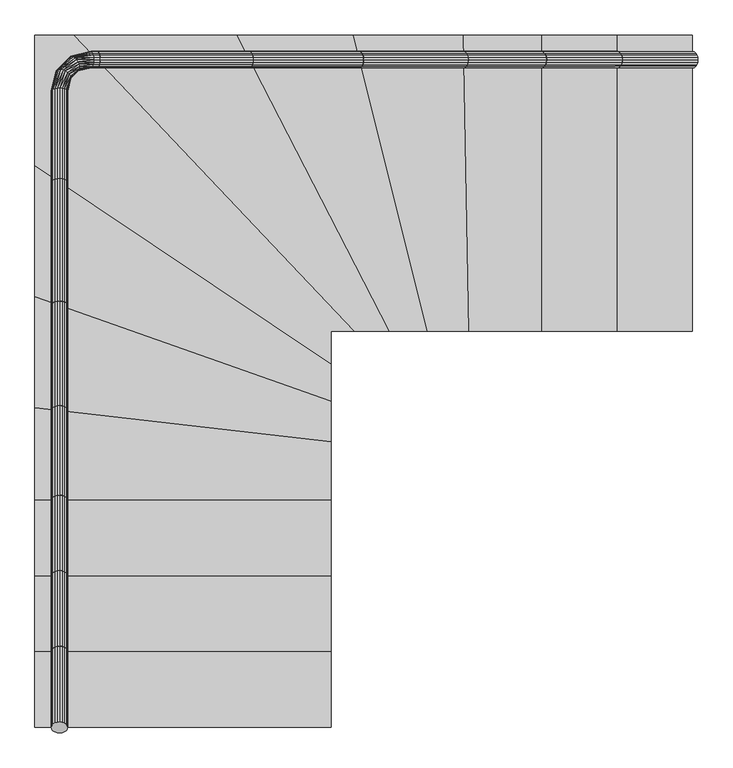
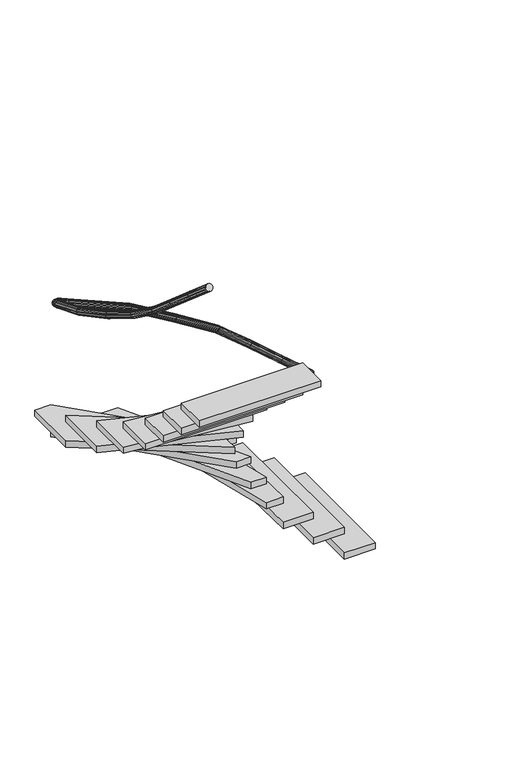
"""IFC4 building model written with IfcOpenShell, lengths in millimetres: stair geometry, 0_3d_modell."""

from ifc_helpers import new_model, si_unit, frame, origin, origin_with_axes, place, context, project, spatial, polyline, outline, extrude, faceted_brep, source, transform, mapped, element, save


def stair_ec7f74a5(model_context):
    return source(origin(), model_context, "Body", "SolidModel", [
        faceted_brep([(51.2235871, 975.7637439, 2650.066583), (50.0, 980.2280824, 2656.7020937), (51.2235871, 984.692421, 2663.3376045), (54.7745751, 988.719759, 2669.3235852), (60.3053687, 991.9158725, 2674.0740863), (67.2745751, 993.9679037, 2677.1240958), (75.0, 994.6749855, 2678.1750575), (82.7254249, 993.9679037, 2677.1240958), (89.6946313, 991.9158725, 2674.0740863), (95.2254249, 988.719759, 2669.3235852), (98.7764129, 984.692421, 2663.3376045), (100.0, 980.2280824, 2656.7020937), (98.7764129, 975.7637439, 2650.066583), (95.2254249, 971.7364059, 2644.0806023), (89.6946313, 968.5402924, 2639.3301012), (82.7254249, 966.4882612, 2636.2800917), (75.0, 965.7811794, 2635.22913), (67.2745751, 966.4882612, 2636.2800917), (60.3053687, 968.5402924, 2639.3301012), (54.7745751, 971.7364059, 2644.0806023), (51.2235871, 711.8708742, 2861.5423857), (50.0, 706.9018591, 2855.2735223), (51.2235871, 701.932844, 2849.004659), (54.7745751, 697.4502308, 2843.3494356), (60.3053687, 693.8928087, 2838.861425), (67.2745751, 691.6088032, 2835.9799448), (75.0, 690.8217885, 2834.9870544), (82.7254249, 691.6088032, 2835.9799448), (89.6946313, 693.8928087, 2838.861425), (95.2254249, 697.4502308, 2843.3494356), (98.7764129, 701.932844, 2849.004659), (100.0, 706.9018591, 2855.2735223), (98.7764129, 711.8708742, 2861.5423857), (95.2254249, 716.3534875, 2867.197609), (89.6946313, 719.9109095, 2871.6856196), (82.7254249, 722.194915, 2874.5670998), (75.0, 722.9819297, 2875.5599903), (67.2745751, 722.194915, 2874.5670998), (60.3053687, 719.9109095, 2871.6856196), (54.7745751, 716.3534875, 2867.197609)], [[[0, 1, 2, 3, 4, 5, 6, 7, 8, 9, 10, 11, 12, 13, 14, 15, 16, 17, 18, 19]], [[20, 21, 22, 23, 24, 25, 26, 27, 28, 29, 30, 31, 32, 33, 34, 35, 36, 37, 38, 39]], [[2, 1, 21, 20]], [[3, 2, 20, 39]], [[4, 3, 39, 38]], [[5, 4, 38, 37]], [[6, 5, 37, 36]], [[7, 6, 36, 35]], [[8, 7, 35, 34]], [[9, 8, 34, 33]], [[10, 9, 33, 32]], [[11, 10, 32, 31]], [[12, 11, 31, 30]], [[13, 12, 30, 29]], [[14, 13, 29, 28]], [[15, 14, 28, 27]], [[16, 15, 27, 26]], [[17, 16, 26, 25]], [[18, 17, 25, 24]], [[19, 18, 24, 23]], [[0, 19, 23, 22]], [[1, 0, 22, 21]]]),
        extrude(outline(polyline([(970.0, 1221.5036957), (900.0, 1221.5036957), (900.0, 1121.5036957), (0.0, 1724.0707938), (0.0, 2121.5036957), (118.0988626, 2121.5036957), (970.0, 1221.5036957)])), frame((0.0, 0.0, 1191.4285714), z_axis=(0.0, 0.0, 1.0), x_axis=(1.0, 0.0, 0.0)), (0.0, 0.0, 1.0), 50.0),
        faceted_brep([(51.2235871, 701.932844, 2849.004659), (50.0, 706.9018591, 2855.2735223), (51.2235871, 711.8708742, 2861.5423857), (54.7745751, 716.3534875, 2867.197609), (60.3053687, 719.9109095, 2871.6856196), (67.2745751, 722.194915, 2874.5670998), (75.0, 722.9819297, 2875.5599903), (82.7254249, 722.194915, 2874.5670998), (89.6946313, 719.9109095, 2871.6856196), (95.2254249, 716.3534875, 2867.197609), (98.7764129, 711.8708742, 2861.5423857), (100.0, 706.9018591, 2855.2735223), (98.7764129, 701.932844, 2849.004659), (95.2254249, 697.4502308, 2843.3494356), (89.6946313, 693.8928087, 2838.861425), (82.7254249, 691.6088032, 2835.9799448), (75.0, 690.8217885, 2834.9870544), (67.2745751, 691.6088032, 2835.9799448), (60.3053687, 693.8928087, 2838.861425), (54.7745751, 697.4502308, 2843.3494356), (51.2235871, 482.1248208, 3059.8945684), (50.0, 476.9018591, 3053.8449509), (51.2235871, 471.6788974, 3047.7953334), (54.7745751, 466.9671956, 3042.3378946), (60.3053687, 463.2279679, 3038.0068466), (67.2745751, 460.8272359, 3035.2261427), (75.0, 460.0, 3034.2679774), (82.7254249, 460.8272359, 3035.2261427), (89.6946313, 463.2279679, 3038.0068466), (95.2254249, 466.9671956, 3042.3378946), (98.7764129, 471.6788974, 3047.7953334), (100.0, 476.9018591, 3053.8449509), (98.7764129, 482.1248208, 3059.8945684), (95.2254249, 486.8365226, 3065.3520072), (89.6946313, 490.5757504, 3069.6830552), (82.7254249, 492.9764824, 3072.4637591), (75.0, 493.8037182, 3073.4219244), (67.2745751, 492.9764824, 3072.4637591), (60.3053687, 490.5757504, 3069.6830552), (54.7745751, 486.8365226, 3065.3520072)], [[[0, 1, 2, 3, 4, 5, 6, 7, 8, 9, 10, 11, 12, 13, 14, 15, 16, 17, 18, 19]], [[20, 21, 22, 23, 24, 25, 26, 27, 28, 29, 30, 31, 32, 33, 34, 35, 36, 37, 38, 39]], [[2, 1, 21, 20]], [[3, 2, 20, 39]], [[4, 3, 39, 38]], [[5, 4, 38, 37]], [[6, 5, 37, 36]], [[7, 6, 36, 35]], [[8, 7, 35, 34]], [[9, 8, 34, 33]], [[10, 9, 33, 32]], [[11, 10, 32, 31]], [[12, 11, 31, 30]], [[13, 12, 30, 29]], [[14, 13, 29, 28]], [[15, 14, 28, 27]], [[16, 15, 27, 26]], [[17, 16, 26, 25]], [[18, 17, 25, 24]], [[19, 18, 24, 23]], [[0, 19, 23, 22]], [[1, 0, 22, 21]]]),
        extrude(outline(polyline([(900.0, 884.9103911), (900.0, 706.9018591), (0.0, 706.9018591), (0.0, 988.8933271), (900.0, 884.9103911)])), frame((0.0, 0.0, 1787.1428571), z_axis=(0.0, 0.0, 1.0), x_axis=(1.0, 0.0, 0.0)), (0.0, 0.0, 1.0), 50.0),
        extrude(outline(polyline([(1077.419675, 1221.5036957), (970.0, 1221.5036957), (118.0988626, 2121.5036957), (613.6390668, 2121.5036957), (1077.419675, 1221.5036957)])), frame((0.0, 0.0, 992.8571429), z_axis=(0.0, 0.0, 1.0), x_axis=(1.0, 0.0, 0.0)), (0.0, 0.0, 1.0), 50.0),
        extrude(outline(polyline([(1192.3186745, 1221.5036957), (1077.419675, 1221.5036957), (613.6390668, 2121.5036957), (967.6813255, 2121.5036957), (1192.3186745, 1221.5036957)])), frame((0.0, 0.0, 794.2857143), z_axis=(0.0, 0.0, 1.0), x_axis=(1.0, 0.0, 0.0)), (0.0, 0.0, 1.0), 50.0),
        extrude(outline(polyline([(900.0, 1121.5036957), (900.0, 1007.5896473), (0.0, 1326.2140709), (0.0, 1724.0707938), (900.0, 1121.5036957)])), frame((0.0, 0.0, 1390.0), z_axis=(0.0, 0.0, 1.0), x_axis=(1.0, 0.0, 0.0)), (0.0, 0.0, 1.0), 50.0),
        extrude(outline(polyline([(900.0, 246.9018591), (900.0, 16.9018591), (0.0, 16.9018591), (0.0, 246.9018591), (900.0, 246.9018591)])), frame((0.0, 0.0, 2382.8571429), z_axis=(0.0, 0.0, 1.0), x_axis=(1.0, 0.0, 0.0)), (0.0, 0.0, 1.0), 50.0),
        faceted_brep([(648.6556288, 2070.2801086, 1855.277549), (652.2874508, 2071.5036957, 1862.4163795), (655.9192729, 2070.2801086, 1869.5552099), (659.1955868, 2066.7291206, 1875.9952419), (661.7956843, 2061.198327, 1881.1060802), (663.4650497, 2054.2291206, 1884.3874404), (664.0402738, 2046.5036957, 1885.51812), (663.4650497, 2038.7782709, 1884.3874404), (661.7956843, 2031.8090644, 1881.1060802), (659.1955868, 2026.2782709, 1875.9952419), (655.9192729, 2022.7272828, 1869.5552099), (652.2874508, 2021.5036957, 1862.4163795), (648.6556288, 2022.7272828, 1855.277549), (645.3793148, 2026.2782709, 1848.8375171), (642.7792174, 2031.8090644, 1843.7266788), (641.109852, 2038.7782709, 1840.4453186), (640.5346279, 2046.5036957, 1839.3146389), (641.109852, 2054.2291206, 1840.4453186), (642.7792174, 2061.198327, 1843.7266788), (645.3793148, 2066.7291206, 1848.8375171), (192.1749264, 2070.2801086, 2068.3613589), (189.0906241, 2071.5036957, 2060.987808), (186.0063217, 2070.2801086, 2053.6142572), (183.2239324, 2066.7291206, 2046.9624808), (181.0158157, 2061.198327, 2041.6836012), (179.5981175, 2054.2291206, 2038.2943519), (179.109612, 2046.5036957, 2037.1264962), (179.5981175, 2038.7782709, 2038.2943519), (181.0158157, 2031.8090644, 2041.6836012), (183.2239324, 2026.2782709, 2046.9624808), (186.0063217, 2022.7272828, 2053.6142572), (189.0906241, 2021.5036957, 2060.987808), (192.1749264, 2022.7272828, 2068.3613589), (194.9573158, 2026.2782709, 2075.0131352), (197.1654325, 2031.8090644, 2080.2920148), (198.5831307, 2038.7782709, 2083.6812642), (199.0716362, 2046.5036957, 2084.8491199), (198.5831307, 2054.2291206, 2083.6812642), (197.1654325, 2061.198327, 2080.2920148), (194.9573158, 2066.7291206, 2075.0131352)], [[[0, 1, 2, 3, 4, 5, 6, 7, 8, 9, 10, 11, 12, 13, 14, 15, 16, 17, 18, 19]], [[20, 21, 22, 23, 24, 25, 26, 27, 28, 29, 30, 31, 32, 33, 34, 35, 36, 37, 38, 39]], [[2, 1, 21, 20]], [[3, 2, 20, 39]], [[4, 3, 39, 38]], [[5, 4, 38, 37]], [[6, 5, 37, 36]], [[7, 6, 36, 35]], [[8, 7, 35, 34]], [[9, 8, 34, 33]], [[10, 9, 33, 32]], [[11, 10, 32, 31]], [[12, 11, 31, 30]], [[13, 12, 30, 29]], [[14, 13, 29, 28]], [[15, 14, 28, 27]], [[16, 15, 27, 26]], [[17, 16, 26, 25]], [[18, 17, 25, 24]], [[19, 18, 24, 23]], [[0, 19, 23, 22]], [[1, 0, 22, 21]]]),
        faceted_brep([(51.2235871, 1670.4655995, 2252.3109173), (50.0, 1673.856869, 2259.5592366), (51.2235871, 1677.2481385, 2266.8075559), (54.7745751, 1680.3074469, 2273.3463592), (60.3053687, 1682.7353278, 2278.5355829), (67.2745751, 1684.2941233, 2281.8672695), (75.0, 1684.8312476, 2283.0152905), (82.7254249, 1684.2941233, 2281.8672695), (89.6946313, 1682.7353278, 2278.5355829), (95.2254249, 1680.3074469, 2273.3463592), (98.7764129, 1677.2481385, 2266.8075559), (100.0, 1673.856869, 2259.5592366), (98.7764129, 1670.4655995, 2252.3109173), (95.2254249, 1667.4062911, 2245.772114), (89.6946313, 1664.9784102, 2240.5828904), (82.7254249, 1663.4196147, 2237.2512037), (75.0, 1662.8824904, 2236.1031827), (67.2745751, 1663.4196147, 2237.2512037), (60.3053687, 1664.9784102, 2240.5828904), (54.7745751, 1667.4062911, 2245.772114), (51.2235871, 1303.6496314, 2465.062536), (50.0, 1299.6620356, 2458.1306652), (51.2235871, 1295.6744399, 2451.1987943), (54.7745751, 1292.0771778, 2444.9454632), (60.3053687, 1289.2223744, 2439.9827916), (67.2745751, 1287.3894778, 2436.7965603), (75.0, 1286.7579047, 2435.6986598), (82.7254249, 1287.3894778, 2436.7965603), (89.6946313, 1289.2223744, 2439.9827916), (95.2254249, 1292.0771778, 2444.9454632), (98.7764129, 1295.6744399, 2451.1987943), (100.0, 1299.6620356, 2458.1306652), (98.7764129, 1303.6496314, 2465.062536), (95.2254249, 1307.2468935, 2471.3158671), (89.6946313, 1310.1016969, 2476.2785387), (82.7254249, 1311.9345935, 2479.46477), (75.0, 1312.5661666, 2480.5626705), (67.2745751, 1311.9345935, 2479.46477), (60.3053687, 1310.1016969, 2476.2785387), (54.7745751, 1307.2468935, 2471.3158671)], [[[0, 1, 2, 3, 4, 5, 6, 7, 8, 9, 10, 11, 12, 13, 14, 15, 16, 17, 18, 19]], [[20, 21, 22, 23, 24, 25, 26, 27, 28, 29, 30, 31, 32, 33, 34, 35, 36, 37, 38, 39]], [[2, 1, 21, 20]], [[3, 2, 20, 39]], [[4, 3, 39, 38]], [[5, 4, 38, 37]], [[6, 5, 37, 36]], [[7, 6, 36, 35]], [[8, 7, 35, 34]], [[9, 8, 34, 33]], [[10, 9, 33, 32]], [[11, 10, 32, 31]], [[12, 11, 31, 30]], [[13, 12, 30, 29]], [[14, 13, 29, 28]], [[15, 14, 28, 27]], [[16, 15, 27, 26]], [[17, 16, 26, 25]], [[18, 17, 25, 24]], [[19, 18, 24, 23]], [[0, 19, 23, 22]], [[1, 0, 22, 21]]]),
        extrude(outline(polyline([(900.0, 476.9018591), (900.0, 246.9018591), (0.0, 246.9018591), (0.0, 476.9018591), (900.0, 476.9018591)])), frame((0.0, 0.0, 2184.2857143), z_axis=(0.0, 0.0, 1.0), x_axis=(1.0, 0.0, 0.0)), (0.0, 0.0, 1.0), 50.0),
        faceted_brep([(1298.5793418, 2070.2801086, 1458.7947987), (1303.2920374, 2071.5036957, 1465.2735223), (1308.004733, 2070.2801086, 1471.7522459), (1312.2561171, 2066.7291206, 1477.5967869), (1315.6300346, 2061.198327, 1482.2350408), (1317.796223, 2054.2291206, 1485.2129832), (1318.5426407, 2046.5036957, 1486.2391122), (1317.796223, 2038.7782709, 1485.2129832), (1315.6300346, 2031.8090644, 1482.2350408), (1312.2561171, 2026.2782709, 1477.5967869), (1308.004733, 2022.7272828, 1471.7522459), (1303.2920374, 2021.5036957, 1465.2735223), (1298.5793418, 2022.7272828, 1458.7947987), (1294.3279577, 2026.2782709, 1452.9502578), (1290.9540401, 2031.8090644, 1448.3120038), (1288.7878517, 2038.7782709, 1445.3340614), (1288.0414341, 2046.5036957, 1444.3079324), (1288.7878517, 2054.2291206, 1445.3340614), (1290.9540401, 2061.198327, 1448.3120038), (1294.3279577, 2066.7291206, 1452.9502578), (990.5652448, 2070.2801086, 1670.6674124), (986.4011046, 2071.5036957, 1663.8449509), (982.2369643, 2070.2801086, 1657.0224894), (978.4804392, 2066.7291206, 1650.867858), (975.4992439, 2061.198327, 1645.9835149), (973.5851987, 2054.2291206, 1642.8475735), (972.9256637, 2046.5036957, 1641.7670018), (973.5851987, 2038.7782709, 1642.8475735), (975.4992439, 2031.8090644, 1645.9835149), (978.4804392, 2026.2782709, 1650.867858), (982.2369643, 2022.7272828, 1657.0224894), (986.4011046, 2021.5036957, 1663.8449509), (990.5652448, 2022.7272828, 1670.6674124), (994.32177, 2026.2782709, 1676.8220438), (997.3029652, 2031.8090644, 1681.7063869), (999.2170104, 2038.7782709, 1684.8423282), (999.8765454, 2046.5036957, 1685.9229), (999.2170104, 2054.2291206, 1684.8423282), (997.3029652, 2061.198327, 1681.7063869), (994.32177, 2066.7291206, 1676.8220438)], [[[0, 1, 2, 3, 4, 5, 6, 7, 8, 9, 10, 11, 12, 13, 14, 15, 16, 17, 18, 19]], [[20, 21, 22, 23, 24, 25, 26, 27, 28, 29, 30, 31, 32, 33, 34, 35, 36, 37, 38, 39]], [[2, 1, 21, 20]], [[3, 2, 20, 39]], [[4, 3, 39, 38]], [[5, 4, 38, 37]], [[6, 5, 37, 36]], [[7, 6, 36, 35]], [[8, 7, 35, 34]], [[9, 8, 34, 33]], [[10, 9, 33, 32]], [[11, 10, 32, 31]], [[12, 11, 31, 30]], [[13, 12, 30, 29]], [[14, 13, 29, 28]], [[15, 14, 28, 27]], [[16, 15, 27, 26]], [[17, 16, 26, 25]], [[18, 17, 25, 24]], [[19, 18, 24, 23]], [[0, 19, 23, 22]], [[1, 0, 22, 21]]]),
        extrude(outline(polyline([(1.2235871, -7.9923214), (0.0, 0.0), (1.2235871, 7.9923214), (4.7745751, 15.2022986), (10.3053687, 20.9241691), (17.2745751, 24.5978359), (25.0, 25.8636953), (32.7254249, 24.5978359), (39.6946313, 20.9241691), (45.2254249, 15.2022986), (48.7764129, 7.9923214), (50.0, 0.0), (48.7764129, -7.9923214), (45.2254249, -15.2022986), (39.6946313, -20.924169), (32.7254249, -24.5978359), (25.0, -25.8636953), (17.2745751, -24.5978359), (10.3053687, -20.924169), (4.7745751, -15.2022986), (1.2235871, -7.9923214)])), frame((50.0, 476.9018591, 3053.8449509), z_axis=(0.0, -0.7569287102856933, 0.6534974579485655), x_axis=(1.0, 0.0, 0.0)), (0.0, 0.0, 1.0), 303.8595272),
        faceted_brep([(1764.7770383, 2070.2801086, 1062.0810477), (1770.0, 2071.5036957, 1068.1306652), (1775.2229617, 2070.2801086, 1074.1802827), (1779.9346635, 2066.7291206, 1079.6377215), (1783.6738913, 2061.198327, 1083.9687694), (1786.0746232, 2054.2291206, 1086.7494734), (1786.9018591, 2046.5036957, 1087.7076387), (1786.0746232, 2038.7782709, 1086.7494734), (1783.6738913, 2031.8090644, 1083.9687694), (1779.9346635, 2026.2782709, 1079.6377215), (1775.2229617, 2022.7272828, 1074.1802827), (1770.0, 2021.5036957, 1068.1306652), (1764.7770383, 2022.7272828, 1062.0810477), (1760.0653365, 2026.2782709, 1056.6236089), (1756.3261087, 2031.8090644, 1052.2925609), (1753.9253768, 2038.7782709, 1049.511857), (1753.0981409, 2046.5036957, 1048.5536917), (1753.9253768, 2054.2291206, 1049.511857), (1756.3261087, 2061.198327, 1052.2925609), (1760.0653365, 2066.7291206, 1056.6236089), (1545.1800436, 2070.2801086, 1272.7887648), (1540.0, 2071.5036957, 1266.7020937), (1534.8199564, 2070.2801086, 1260.6154227), (1530.1469716, 2066.7291206, 1255.1245574), (1526.4384698, 2061.198327, 1250.7669821), (1524.0574652, 2054.2291206, 1247.9692465), (1523.2370268, 2046.5036957, 1247.0052125), (1524.0574652, 2038.7782709, 1247.9692465), (1526.4384698, 2031.8090644, 1250.7669821), (1530.1469716, 2026.2782709, 1255.1245574), (1534.8199564, 2022.7272828, 1260.6154227), (1540.0, 2021.5036957, 1266.7020937), (1545.1800436, 2022.7272828, 1272.7887648), (1549.8530284, 2026.2782709, 1278.2796301), (1553.5615302, 2031.8090644, 1282.6372054), (1555.9425348, 2038.7782709, 1285.434941), (1556.7629732, 2046.5036957, 1286.398975), (1555.9425348, 2054.2291206, 1285.434941), (1553.5615302, 2061.198327, 1282.6372054), (1549.8530284, 2066.7291206, 1278.2796301)], [[[0, 1, 2, 3, 4, 5, 6, 7, 8, 9, 10, 11, 12, 13, 14, 15, 16, 17, 18, 19]], [[20, 21, 22, 23, 24, 25, 26, 27, 28, 29, 30, 31, 32, 33, 34, 35, 36, 37, 38, 39]], [[2, 1, 21, 20]], [[3, 2, 20, 39]], [[4, 3, 39, 38]], [[5, 4, 38, 37]], [[6, 5, 37, 36]], [[7, 6, 36, 35]], [[8, 7, 35, 34]], [[9, 8, 34, 33]], [[10, 9, 33, 32]], [[11, 10, 32, 31]], [[12, 11, 31, 30]], [[13, 12, 30, 29]], [[14, 13, 29, 28]], [[15, 14, 28, 27]], [[16, 15, 27, 26]], [[17, 16, 26, 25]], [[18, 17, 25, 24]], [[19, 18, 24, 23]], [[0, 19, 23, 22]], [[1, 0, 22, 21]]]),
        faceted_brep([(51.2235871, 1295.6744399, 2451.1987943), (50.0, 1299.6620356, 2458.1306652), (51.2235871, 1303.6496314, 2465.062536), (54.7745751, 1307.2468935, 2471.3158671), (60.3053687, 1310.1016969, 2476.2785387), (67.2745751, 1311.9345935, 2479.46477), (75.0, 1312.5661666, 2480.5626705), (82.7254249, 1311.9345935, 2479.46477), (89.6946313, 1310.1016969, 2476.2785387), (95.2254249, 1307.2468935, 2471.3158671), (98.7764129, 1303.6496314, 2465.062536), (100.0, 1299.6620356, 2458.1306652), (98.7764129, 1295.6744399, 2451.1987943), (95.2254249, 1292.0771778, 2444.9454632), (89.6946313, 1289.2223744, 2439.9827916), (82.7254249, 1287.3894778, 2436.7965603), (75.0, 1286.7579047, 2435.6986598), (67.2745751, 1287.3894778, 2436.7965603), (60.3053687, 1289.2223744, 2439.9827916), (54.7745751, 1292.0771778, 2444.9454632), (51.2235871, 984.692421, 2663.3376045), (50.0, 980.2280824, 2656.7020937), (51.2235871, 975.7637439, 2650.066583), (54.7745751, 971.7364059, 2644.0806023), (60.3053687, 968.5402924, 2639.3301012), (67.2745751, 966.4882612, 2636.2800917), (75.0, 965.7811794, 2635.22913), (82.7254249, 966.4882612, 2636.2800917), (89.6946313, 968.5402924, 2639.3301012), (95.2254249, 971.7364059, 2644.0806023), (98.7764129, 975.7637439, 2650.066583), (100.0, 980.2280824, 2656.7020937), (98.7764129, 984.692421, 2663.3376045), (95.2254249, 988.719759, 2669.3235852), (89.6946313, 991.9158725, 2674.0740863), (82.7254249, 993.9679037, 2677.1240958), (75.0, 994.6749855, 2678.1750575), (67.2745751, 993.9679037, 2677.1240958), (60.3053687, 991.9158725, 2674.0740863), (54.7745751, 988.719759, 2669.3235852)], [[[0, 1, 2, 3, 4, 5, 6, 7, 8, 9, 10, 11, 12, 13, 14, 15, 16, 17, 18, 19]], [[20, 21, 22, 23, 24, 25, 26, 27, 28, 29, 30, 31, 32, 33, 34, 35, 36, 37, 38, 39]], [[2, 1, 21, 20]], [[3, 2, 20, 39]], [[4, 3, 39, 38]], [[5, 4, 38, 37]], [[6, 5, 37, 36]], [[7, 6, 36, 35]], [[8, 7, 35, 34]], [[9, 8, 34, 33]], [[10, 9, 33, 32]], [[11, 10, 32, 31]], [[12, 11, 31, 30]], [[13, 12, 30, 29]], [[14, 13, 29, 28]], [[15, 14, 28, 27]], [[16, 15, 27, 26]], [[17, 16, 26, 25]], [[18, 17, 25, 24]], [[19, 18, 24, 23]], [[0, 19, 23, 22]], [[1, 0, 22, 21]]]),
        faceted_brep([(1534.8199564, 2070.2801086, 1260.6154227), (1540.0, 2071.5036957, 1266.7020937), (1545.1800436, 2070.2801086, 1272.7887648), (1549.8530284, 2066.7291206, 1278.2796301), (1553.5615302, 2061.198327, 1282.6372054), (1555.9425348, 2054.2291206, 1285.434941), (1556.7629732, 2046.5036957, 1286.398975), (1555.9425348, 2038.7782709, 1285.434941), (1553.5615302, 2031.8090644, 1282.6372054), (1549.8530284, 2026.2782709, 1278.2796301), (1545.1800436, 2022.7272828, 1272.7887648), (1540.0, 2021.5036957, 1266.7020937), (1534.8199564, 2022.7272828, 1260.6154227), (1530.1469716, 2026.2782709, 1255.1245574), (1526.4384698, 2031.8090644, 1250.7669821), (1524.0574652, 2038.7782709, 1247.9692465), (1523.2370268, 2046.5036957, 1247.0052125), (1524.0574652, 2054.2291206, 1247.9692465), (1526.4384698, 2061.198327, 1250.7669821), (1530.1469716, 2066.7291206, 1255.1245574), (1308.004733, 2070.2801086, 1471.7522459), (1303.2920374, 2071.5036957, 1465.2735223), (1298.5793418, 2070.2801086, 1458.7947987), (1294.3279577, 2066.7291206, 1452.9502578), (1290.9540401, 2061.198327, 1448.3120038), (1288.7878517, 2054.2291206, 1445.3340614), (1288.0414341, 2046.5036957, 1444.3079324), (1288.7878517, 2038.7782709, 1445.3340614), (1290.9540401, 2031.8090644, 1448.3120038), (1294.3279577, 2026.2782709, 1452.9502578), (1298.5793418, 2022.7272828, 1458.7947987), (1303.2920374, 2021.5036957, 1465.2735223), (1308.004733, 2022.7272828, 1471.7522459), (1312.2561171, 2026.2782709, 1477.5967869), (1315.6300346, 2031.8090644, 1482.2350408), (1317.796223, 2038.7782709, 1485.2129832), (1318.5426407, 2046.5036957, 1486.2391122), (1317.796223, 2054.2291206, 1485.2129832), (1315.6300346, 2061.198327, 1482.2350408), (1312.2561171, 2066.7291206, 1477.5967869)], [[[0, 1, 2, 3, 4, 5, 6, 7, 8, 9, 10, 11, 12, 13, 14, 15, 16, 17, 18, 19]], [[20, 21, 22, 23, 24, 25, 26, 27, 28, 29, 30, 31, 32, 33, 34, 35, 36, 37, 38, 39]], [[2, 1, 21, 20]], [[3, 2, 20, 39]], [[4, 3, 39, 38]], [[5, 4, 38, 37]], [[6, 5, 37, 36]], [[7, 6, 36, 35]], [[8, 7, 35, 34]], [[9, 8, 34, 33]], [[10, 9, 33, 32]], [[11, 10, 32, 31]], [[12, 11, 31, 30]], [[13, 12, 30, 29]], [[14, 13, 29, 28]], [[15, 14, 28, 27]], [[16, 15, 27, 26]], [[17, 16, 26, 25]], [[18, 17, 25, 24]], [[19, 18, 24, 23]], [[0, 19, 23, 22]], [[1, 0, 22, 21]]]),
        extrude(outline(polyline([(1.2235871, -7.9923214), (0.0, 0.0), (1.2235871, 7.9923214), (4.7745751, 15.2022986), (10.3053687, 20.9241691), (17.2745751, 24.5978359), (25.0, 25.8636953), (32.7254248, 24.5978359), (39.6946313, 20.9241691), (45.2254248, 15.2022986), (48.7764129, 7.9923214), (50.0, 0.0), (48.7764129, -7.9923214), (45.2254248, -15.2022986), (39.6946313, -20.9241691), (32.7254248, -24.5978359), (25.0, -25.8636953), (17.2745751, -24.5978359), (10.3053687, -20.9241691), (4.7745751, -15.2022986), (1.2235871, -7.9923214)])), frame((2000.0, 2071.5036957, 869.5592366), z_axis=(-0.7569287102857639, 0.0, 0.6534974579484836), x_axis=(0.0, -1.0, 0.0)), (0.0, 0.0, 1.0), 303.8595272),
        faceted_brep([(186.0063217, 2070.2801086, 2053.6142572), (189.0906241, 2071.5036957, 2060.987808), (192.1749264, 2070.2801086, 2068.3613589), (194.9573158, 2066.7291206, 2075.0131352), (197.1654325, 2061.198327, 2080.2920148), (198.5831307, 2054.2291206, 2083.6812642), (199.0716362, 2046.5036957, 2084.8491199), (198.5831307, 2038.7782709, 2083.6812642), (197.1654325, 2031.8090644, 2080.2920148), (194.9573158, 2026.2782709, 2075.0131352), (192.1749264, 2022.7272828, 2068.3613589), (189.0906241, 2021.5036957, 2060.987808), (186.0063217, 2022.7272828, 2053.6142572), (183.2239324, 2026.2782709, 2046.9624808), (181.0158157, 2031.8090644, 2041.6836012), (179.5981175, 2038.7782709, 2038.2943519), (179.109612, 2046.5036957, 2037.1264962), (179.5981175, 2054.2291206, 2038.2943519), (181.0158157, 2061.198327, 2041.6836012), (183.2239324, 2066.7291206, 2046.9624808), (51.2235871, 1677.2481385, 2266.8075559), (50.0, 1673.856869, 2259.5592366), (51.2235871, 1670.4655995, 2252.3109173), (54.7745751, 1667.4062911, 2245.772114), (60.3053687, 1664.9784102, 2240.5828904), (67.2745751, 1663.4196147, 2237.2512037), (75.0, 1662.8824904, 2236.1031827), (82.7254249, 1663.4196147, 2237.2512037), (89.6946313, 1664.9784102, 2240.5828904), (95.2254249, 1667.4062911, 2245.772114), (98.7764129, 1670.4655995, 2252.3109173), (100.0, 1673.856869, 2259.5592366), (98.7764129, 1677.2481385, 2266.8075559), (95.2254249, 1680.3074469, 2273.3463592), (89.6946313, 1682.7353278, 2278.5355829), (82.7254249, 1684.2941233, 2281.8672695), (75.0, 1684.8312476, 2283.0152905), (67.2745751, 1684.2941233, 2281.8672695), (60.3053687, 1682.7353278, 2278.5355829), (54.7745751, 1680.3074469, 2273.3463592), (170.7900373, 2071.5036957, 2068.4537913), (173.8090484, 2070.2801086, 2075.8539787), (176.5325377, 2066.7291206, 2082.5297841), (178.693911, 2061.198327, 2087.8277333), (180.0815981, 2054.2291206, 2091.2292261), (180.5597625, 2046.5036957, 2092.4013006), (180.0815981, 2038.7782709, 2091.2292261), (178.693911, 2031.8090644, 2087.8277333), (176.5325377, 2026.2782709, 2082.5297841), (173.8090484, 2022.7272828, 2075.8539787), (170.7900373, 2021.5036957, 2068.4537913), (167.7710262, 2022.7272828, 2061.053604), (165.0475369, 2026.2782709, 2054.3777985), (162.8861636, 2031.8090644, 2049.0798493), (161.4984765, 2038.7782709, 2045.6783565), (161.0203121, 2046.5036957, 2044.506282), (161.4984765, 2054.2291206, 2045.6783565), (162.8861636, 2061.198327, 2049.0798493), (165.0475369, 2066.7291206, 2054.3777985), (167.7710262, 2070.2801086, 2061.053604), (108.2229833, 2056.4792109, 2093.9682441), (112.2067376, 2057.2618667, 2100.9604911), (116.9740597, 2055.8204705, 2107.2682883), (122.058291, 2052.2961161, 2112.2741844), (126.9617515, 2047.0337921, 2115.4881676), (131.2044563, 2040.5486112, 2116.5956307), (134.3710999, 2033.4753883, 2115.4881676), (136.1517092, 2026.5064996, 2112.2741844), (136.3719857, 2020.3241085, 2107.2682883), (135.0103672, 2015.5333905, 2100.9604911), (132.2001384, 2012.6032946, 2093.9682441), (128.2163841, 2011.8206388, 2086.9759971), (123.449062, 2013.262035, 2080.6681999), (118.3648307, 2016.7863894, 2075.6623037), (113.4613702, 2022.0487134, 2072.4483206), (109.2186654, 2028.5338943, 2071.3408574), (106.0520218, 2035.6071172, 2072.4483206), (104.2714126, 2042.5760059, 2075.6623037), (104.0511361, 2048.758397, 2080.6681999), (105.4127546, 2053.549115, 2086.9759971), (65.0244848, 2013.2807124, 2121.0971401), (67.9545808, 2016.0909411, 2128.0893871), (72.7452987, 2017.4525596, 2134.3971843), (78.9276898, 2017.2322831, 2139.4030804), (85.8965785, 2015.4516739, 2142.6170636), (92.9698015, 2012.2850303, 2143.7245267), (99.4549823, 2008.0423255, 2142.6170636), (104.7173064, 2003.138865, 2139.4030804), (108.2416607, 1998.0546337, 2134.3971843), (109.6830569, 1993.2873116, 2128.0893871), (108.9004011, 1989.3035573, 2121.0971401), (105.9703052, 1986.4933285, 2114.1048931), (101.1795872, 1985.1317101, 2107.7970959), (94.9971961, 1985.3519865, 2102.7911997), (88.0283074, 1987.1325958, 2099.5772166), (80.9550845, 1990.2992394, 2098.4697534), (74.4699036, 1994.5419442, 2099.5772166), (69.2075796, 1999.4454047, 2102.7911997), (65.6832253, 2004.529636, 2107.7970959), (64.241829, 2009.2969581, 2114.1048931), (50.0, 1950.7136584, 2146.6115929), (51.2235871, 1953.7326696, 2154.0117802), (54.7745751, 1956.4561588, 2160.6875857), (60.3053687, 1958.6175321, 2165.9855349), (67.2745751, 1960.0052192, 2169.3870277), (75.0, 1960.4833836, 2170.5591022), (82.7254249, 1960.0052192, 2169.3870277), (89.6946313, 1958.6175321, 2165.9855349), (95.2254249, 1956.4561588, 2160.6875857), (98.7764129, 1953.7326696, 2154.0117802), (100.0, 1950.7136584, 2146.6115929), (98.7764129, 1947.6946473, 2139.2114055), (95.2254249, 1944.971158, 2132.5356001), (89.6946313, 1942.8097847, 2127.2376509), (82.7254249, 1941.4220976, 2123.8361581), (75.0, 1940.9439332, 2122.6640835), (67.2745751, 1941.4220976, 2123.8361581), (60.3053687, 1942.8097847, 2127.2376509), (54.7745751, 1944.971158, 2132.5356001), (51.2235871, 1947.6946473, 2139.2114055)], [[[0, 1, 2, 3, 4, 5, 6, 7, 8, 9, 10, 11, 12, 13, 14, 15, 16, 17, 18, 19]], [[20, 21, 22, 23, 24, 25, 26, 27, 28, 29, 30, 31, 32, 33, 34, 35, 36, 37, 38, 39]], [[2, 1, 40, 41]], [[3, 2, 41, 42]], [[4, 3, 42, 43]], [[5, 4, 43, 44]], [[6, 5, 44, 45]], [[7, 6, 45, 46]], [[8, 7, 46, 47]], [[9, 8, 47, 48]], [[10, 9, 48, 49]], [[11, 10, 49, 50]], [[12, 11, 50, 51]], [[13, 12, 51, 52]], [[14, 13, 52, 53]], [[15, 14, 53, 54]], [[16, 15, 54, 55]], [[17, 16, 55, 56]], [[18, 17, 56, 57]], [[19, 18, 57, 58]], [[0, 19, 58, 59]], [[1, 0, 59, 40]], [[41, 40, 60]], [[61, 41, 60]], [[42, 41, 61]], [[62, 42, 61]], [[43, 42, 62]], [[63, 43, 62]], [[44, 43, 63]], [[64, 44, 63]], [[45, 44, 64]], [[65, 45, 64]], [[46, 45, 65]], [[66, 46, 65]], [[47, 46, 66]], [[67, 47, 66]], [[48, 47, 67]], [[68, 48, 67]], [[49, 48, 68]], [[69, 49, 68]], [[50, 49, 69]], [[70, 50, 69]], [[51, 50, 70]], [[71, 51, 70]], [[52, 51, 71]], [[72, 52, 71]], [[53, 52, 72]], [[73, 53, 72]], [[54, 53, 73]], [[74, 54, 73]], [[55, 54, 74]], [[75, 55, 74]], [[56, 55, 75]], [[76, 56, 75]], [[57, 56, 76]], [[77, 57, 76]], [[58, 57, 77]], [[78, 58, 77]], [[59, 58, 78]], [[79, 59, 78]], [[40, 59, 79]], [[60, 40, 79]], [[61, 60, 80]], [[81, 61, 80]], [[62, 61, 81]], [[82, 62, 81]], [[63, 62, 82]], [[83, 63, 82]], [[64, 63, 83]], [[84, 64, 83]], [[65, 64, 84]], [[85, 65, 84]], [[66, 65, 85]], [[86, 66, 85]], [[67, 66, 86]], [[87, 67, 86]], [[68, 67, 87]], [[88, 68, 87]], [[69, 68, 88]], [[89, 69, 88]], [[70, 69, 89]], [[90, 70, 89]], [[71, 70, 90]], [[91, 71, 90]], [[72, 71, 91]], [[92, 72, 91]], [[73, 72, 92]], [[93, 73, 92]], [[74, 73, 93]], [[94, 74, 93]], [[75, 74, 94]], [[95, 75, 94]], [[76, 75, 95]], [[96, 76, 95]], [[77, 76, 96]], [[97, 77, 96]], [[78, 77, 97]], [[98, 78, 97]], [[79, 78, 98]], [[99, 79, 98]], [[60, 79, 99]], [[80, 60, 99]], [[81, 80, 100]], [[101, 81, 100]], [[82, 81, 101]], [[102, 82, 101]], [[83, 82, 102]], [[103, 83, 102]], [[84, 83, 103]], [[104, 84, 103]], [[85, 84, 104]], [[105, 85, 104]], [[86, 85, 105]], [[106, 86, 105]], [[87, 86, 106]], [[107, 87, 106]], [[88, 87, 107]], [[108, 88, 107]], [[89, 88, 108]], [[109, 89, 108]], [[90, 89, 109]], [[110, 90, 109]], [[91, 90, 110]], [[111, 91, 110]], [[92, 91, 111]], [[112, 92, 111]], [[93, 92, 112]], [[113, 93, 112]], [[94, 93, 113]], [[114, 94, 113]], [[95, 94, 114]], [[115, 95, 114]], [[96, 95, 115]], [[116, 96, 115]], [[97, 96, 116]], [[117, 97, 116]], [[98, 97, 117]], [[118, 98, 117]], [[99, 98, 118]], [[119, 99, 118]], [[80, 99, 119]], [[100, 80, 119]], [[101, 100, 21, 20]], [[102, 101, 20, 39]], [[103, 102, 39, 38]], [[104, 103, 38, 37]], [[105, 104, 37, 36]], [[106, 105, 36, 35]], [[107, 106, 35, 34]], [[108, 107, 34, 33]], [[109, 108, 33, 32]], [[110, 109, 32, 31]], [[111, 110, 31, 30]], [[112, 111, 30, 29]], [[113, 112, 29, 28]], [[114, 113, 28, 27]], [[115, 114, 27, 26]], [[116, 115, 26, 25]], [[117, 116, 25, 24]], [[118, 117, 24, 23]], [[119, 118, 23, 22]], [[100, 119, 22, 21]]]),
        extrude(outline(polyline([(900.0, 706.9018591), (900.0, 476.9018591), (0.0, 476.9018591), (0.0, 706.9018591), (900.0, 706.9018591)])), frame((0.0, 0.0, 1985.7142857), z_axis=(0.0, 0.0, 1.0), x_axis=(1.0, 0.0, 0.0)), (0.0, 0.0, 1.0), 50.0),
        extrude(outline(polyline([(900.0, 1007.5896473), (900.0, 884.9103911), (0.0, 988.8933271), (0.0, 1326.2140709), (900.0, 1007.5896473)])), frame((0.0, 0.0, 1588.5714286), z_axis=(0.0, 0.0, 1.0), x_axis=(1.0, 0.0, 0.0)), (0.0, 0.0, 1.0), 50.0),
        extrude(outline(polyline([(2000.0, 1221.5036957), (1770.0, 1221.5036957), (1770.0, 2121.5036957), (2000.0, 2121.5036957), (2000.0, 1221.5036957)])), origin_with_axes(), (0.0, 0.0, 1.0), 50.0),
        extrude(outline(polyline([(1540.0, 1221.5036957), (1318.0495551, 1221.5036957), (1301.9504449, 2121.5036957), (1540.0, 2121.5036957), (1540.0, 1221.5036957)])), frame((0.0, 0.0, 397.1428571), z_axis=(0.0, 0.0, 1.0), x_axis=(1.0, 0.0, 0.0)), (0.0, 0.0, 1.0), 50.0),
        extrude(outline(polyline([(1770.0, 1221.5036957), (1540.0, 1221.5036957), (1540.0, 2121.5036957), (1770.0, 2121.5036957), (1770.0, 1221.5036957)])), frame((0.0, 0.0, 198.5714286), z_axis=(0.0, 0.0, 1.0), x_axis=(1.0, 0.0, 0.0)), (0.0, 0.0, 1.0), 50.0),
        extrude(outline(polyline([(1318.0495551, 1221.5036957), (1192.3186745, 1221.5036957), (967.6813255, 2121.5036957), (1301.9504449, 2121.5036957), (1318.0495551, 1221.5036957)])), frame((0.0, 0.0, 595.7142857), z_axis=(0.0, 0.0, 1.0), x_axis=(1.0, 0.0, 0.0)), (0.0, 0.0, 1.0), 50.0),
        extrude(outline(polyline([(1.2235871, -7.9923214), (0.0, 0.0), (1.2235871, 7.9923214), (4.7745751, 15.2022986), (10.3053687, 20.924169), (17.2745751, 24.5978359), (25.0, 25.8636953), (32.7254249, 24.5978359), (39.6946313, 20.924169), (45.2254249, 15.2022986), (48.7764129, 7.9923214), (50.0, 0.0), (48.7764129, -7.9923214), (45.2254249, -15.2022986), (39.6946313, -20.924169), (32.7254249, -24.597836), (25.0, -25.8636953), (17.2745751, -24.597836), (10.3053687, -20.924169), (4.7745751, -15.2022986), (1.2235871, -7.9923214)])), frame((50.0, 246.9018591, 3252.4163795), z_axis=(0.0, -0.7569287102857001, 0.6534974579485575), x_axis=(1.0, 0.0, 0.0)), (0.0, 0.0, 1.0), 303.8595272),
        faceted_brep([(982.2369643, 2070.2801086, 1657.0224894), (986.4011046, 2071.5036957, 1663.8449509), (990.5652448, 2070.2801086, 1670.6674124), (994.32177, 2066.7291206, 1676.8220438), (997.3029652, 2061.198327, 1681.7063869), (999.2170104, 2054.2291206, 1684.8423282), (999.8765454, 2046.5036957, 1685.9229), (999.2170104, 2038.7782709, 1684.8423282), (997.3029652, 2031.8090644, 1681.7063869), (994.32177, 2026.2782709, 1676.8220438), (990.5652448, 2022.7272828, 1670.6674124), (986.4011046, 2021.5036957, 1663.8449509), (982.2369643, 2022.7272828, 1657.0224894), (978.4804392, 2026.2782709, 1650.867858), (975.4992439, 2031.8090644, 1645.9835149), (973.5851987, 2038.7782709, 1642.8475735), (972.9256637, 2046.5036957, 1641.7670018), (973.5851987, 2054.2291206, 1642.8475735), (975.4992439, 2061.198327, 1645.9835149), (978.4804392, 2066.7291206, 1650.867858), (655.9192729, 2070.2801086, 1869.5552099), (652.2874508, 2071.5036957, 1862.4163795), (648.6556288, 2070.2801086, 1855.277549), (645.3793148, 2066.7291206, 1848.8375171), (642.7792174, 2061.198327, 1843.7266788), (641.109852, 2054.2291206, 1840.4453186), (640.5346279, 2046.5036957, 1839.3146389), (641.109852, 2038.7782709, 1840.4453186), (642.7792174, 2031.8090644, 1843.7266788), (645.3793148, 2026.2782709, 1848.8375171), (648.6556288, 2022.7272828, 1855.277549), (652.2874508, 2021.5036957, 1862.4163795), (655.9192729, 2022.7272828, 1869.5552099), (659.1955868, 2026.2782709, 1875.9952419), (661.7956843, 2031.8090644, 1881.1060802), (663.4650497, 2038.7782709, 1884.3874404), (664.0402738, 2046.5036957, 1885.51812), (663.4650497, 2054.2291206, 1884.3874404), (661.7956843, 2061.198327, 1881.1060802), (659.1955868, 2066.7291206, 1875.9952419)], [[[0, 1, 2, 3, 4, 5, 6, 7, 8, 9, 10, 11, 12, 13, 14, 15, 16, 17, 18, 19]], [[20, 21, 22, 23, 24, 25, 26, 27, 28, 29, 30, 31, 32, 33, 34, 35, 36, 37, 38, 39]], [[2, 1, 21, 20]], [[3, 2, 20, 39]], [[4, 3, 39, 38]], [[5, 4, 38, 37]], [[6, 5, 37, 36]], [[7, 6, 36, 35]], [[8, 7, 35, 34]], [[9, 8, 34, 33]], [[10, 9, 33, 32]], [[11, 10, 32, 31]], [[12, 11, 31, 30]], [[13, 12, 30, 29]], [[14, 13, 29, 28]], [[15, 14, 28, 27]], [[16, 15, 27, 26]], [[17, 16, 26, 25]], [[18, 17, 25, 24]], [[19, 18, 24, 23]], [[0, 19, 23, 22]], [[1, 0, 22, 21]]]),
    ])


if __name__ == "__main__":
    model = new_model("IFC4")
    model_context = context("Model", 3, world=origin())
    ifc_project = project(units=[si_unit("LENGTHUNIT", "METRE", prefix="MILLI")], contexts=[model_context])
    site = spatial("IfcSite", under=ifc_project)
    building = spatial("IfcBuilding", under=site)
    placement = place(None, origin())
    stair_shape = stair_ec7f74a5(model_context)
    element("IfcStair", 1, ObjectType="0_3d_modell", at=placement, inside=building, context=model_context, shape_type="MappedRepresentation", body=[
        mapped(stair_shape, transform((0.0, 0.0, 0.0), x_axis=(1.0, 0.0, 0.0), y_axis=(0.0, 1.0, 0.0), z_axis=(0.0, 0.0, 1.0))),
    ])
    save(model, "model.ifc")

# Revit data of these elements
# Element 1 (IfcStair, "0_3d_modell")
#   Materials on its faces: "*1", "weiss"
# Materials
#   "*1": class "Unassigned", colour RGB 175 175 175, transparency 0
#   "weiss": class "Unassigned", colour RGB 255 255 255, transparency 0
